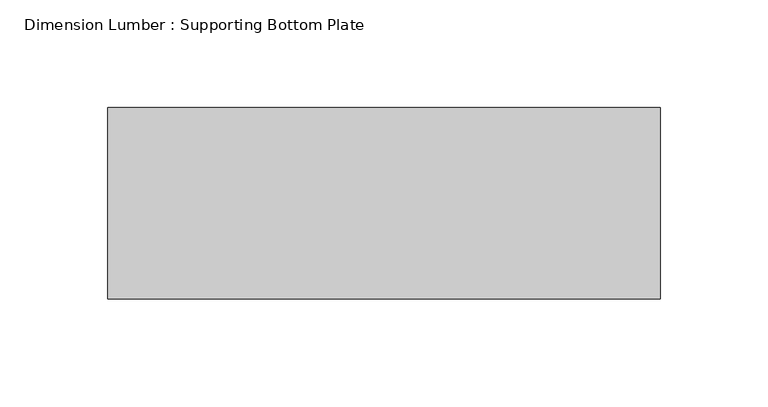
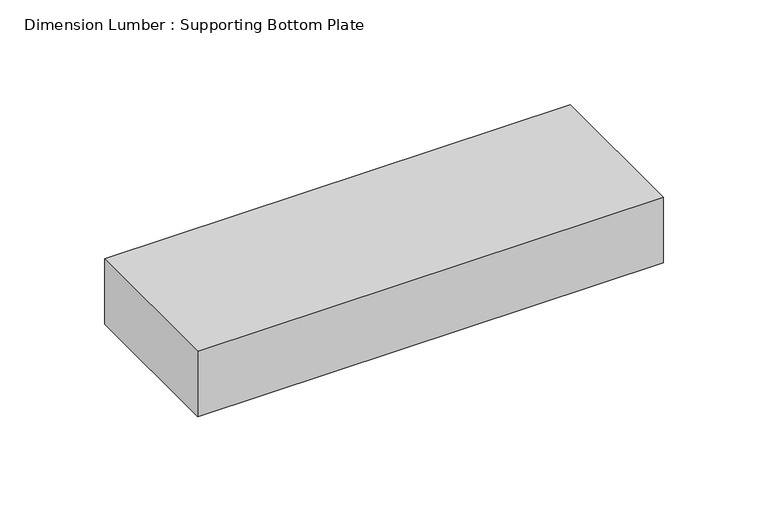
"""IFC4 building model written with IfcOpenShell, lengths in millimetres: beam geometry, Dimension Lumber : Supporting Bottom Plate."""

from ifc_helpers import new_model, si_unit, frame, origin, place, context, project, spatial, polyline, outline, extrude, source, transform, mapped, element, save


def dimension_lumber_supporting_bottom_plate_90e85d83(model_context):
    return source(origin(), model_context, "Body", "SweptSolid", [
        extrude(outline(polyline([(128.190625, 44.45), (128.190625, -44.45), (-128.190625, -44.45), (-128.190625, 44.45), (128.190625, 44.45)])), frame((0.0, 0.0, -19.05), z_axis=(0.0, 0.0, 1.0), x_axis=(1.0, 0.0, 0.0)), (0.0, 0.0, 1.0), 38.1),
    ])


if __name__ == "__main__":
    model = new_model("IFC4")
    model_context = context("Model", 3, world=origin())
    ifc_project = project(units=[si_unit("LENGTHUNIT", "METRE", prefix="MILLI")], contexts=[model_context])
    site = spatial("IfcSite", under=ifc_project)
    building = spatial("IfcBuilding", under=site)
    placement = place(None, origin())
    dimension_lumber_supporting_bottom_plate_shape = dimension_lumber_supporting_bottom_plate_90e85d83(model_context)
    element("IfcBeam", 1, ObjectType="Dimension Lumber : Supporting Bottom Plate", at=placement, inside=building, context=model_context, shape_type="MappedRepresentation", body=[
        mapped(dimension_lumber_supporting_bottom_plate_shape, transform((0.0, 0.0, 0.0), x_axis=(1.0, 0.0, 0.0), y_axis=(0.0, 1.0, 0.0), z_axis=(0.0, 0.0, 1.0))),
    ])
    save(model, "model.ifc")

# Revit data of these elements
# Type "Dimension Lumber : Supporting Bottom Plate"
#   Assembly Code = "B10"
#   A = 0.0364583 SF
#   Length [instance default] = 5' - 0"
#   b = 0' - 3 1/2"
#   d = 0' - 1 1/2"
#   Structural Material [instance default] = Softwood, Lumber
# Element 1 (IfcBeam, "Dimension Lumber : Supporting Bottom Plate")
#   Structural Material = Douglas Fir #2
#   Materials on its faces: "Douglas Fir #2"
# Materials
#   "Softwood, Lumber": class "Wood", colour RGB 223 192 134, transparency 0, Description = "Pinus Echinata", Cost = 0
#   "Douglas Fir #2": class "Wood", colour RGB 223 192 134, transparency 0, Description = "Pinus Echinata", Cost = 0
